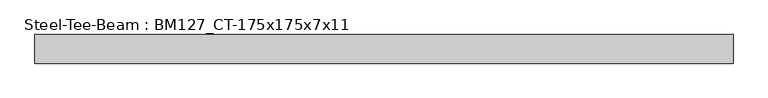
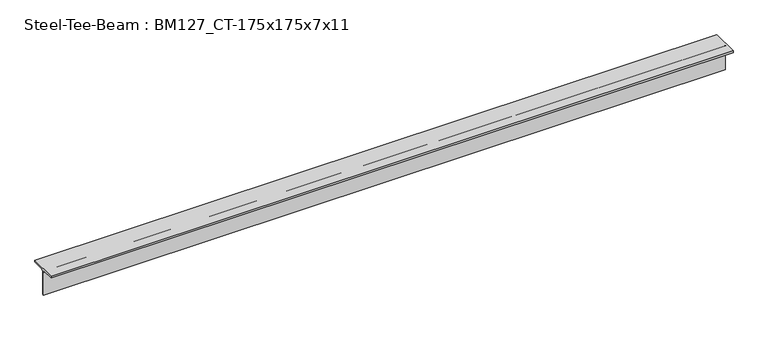
"""IFC4 building model written with IfcOpenShell, lengths in millimetres: beam geometry, Steel-Tee-Beam : BM127_CT-175x175x7x11."""

import ifcopenshell
import ifcopenshell.guid

model = None  # the IFC model being written
_history = None  # IfcOwnerHistory: only IFC2X3 demands one
_inside = {}  # id of a spatial element -> (the spatial element, [elements in it])
_under = {}  # id of a project, library or spatial element -> (it, [spatial elements below it])
_declared = {}  # id of a project -> (the project, [libraries it declares])
_typed = {}  # id of a type object -> (the type object, [elements of that type])
_made_of = {}  # id of a material, layer set ... -> (it, [elements and type objects made of it])


def new_model(schema):
    """Start an empty IFC model of exactly this schema.

    Asked for "IFC4X3", IfcOpenShell would pick the latest addendum, in which some entities
    have other attributes; the version numbers below select the first issue.
    IFC2X3 requires an IfcOwnerHistory on every rooted entity: one is made here for all.
    """
    global model, _history
    if schema == "IFC4X3":
        model = ifcopenshell.file(schema_version=(4, 3, 0, 0))
    else:
        model = ifcopenshell.file(schema=schema)
    _inside.clear()
    _under.clear()
    _declared.clear()
    _typed.clear()
    _made_of.clear()
    _history = None
    if model.schema == "IFC2X3":
        org = make("IfcOrganization", Name="unknown")
        user = make(
            "IfcPersonAndOrganization",
            ThePerson=make("IfcPerson", FamilyName="unknown"),
            TheOrganization=org,
        )
        app = make(
            "IfcApplication",
            ApplicationDeveloper=org,
            Version="unknown",
            ApplicationFullName="unknown",
            ApplicationIdentifier="unknown",
        )
        _history = make(
            "IfcOwnerHistory",
            OwningUser=user,
            OwningApplication=app,
            ChangeAction="ADDED",
            CreationDate=0,
        )
    return model


def make(cls, **values):
    """One entity of the class cls with the attributes given. An attribute that is None is left unset."""
    return model.create_entity(
        cls, **{name: value for name, value in values.items() if value is not None}
    )


def rooted(cls, **values):
    """An entity with a GlobalId (a new one), such as an element, a storey or a relation."""
    return make(cls, GlobalId=ifcopenshell.guid.new(), OwnerHistory=_history, **values)


def si_unit(unit_type, name, prefix=None):
    """IfcSIUnit, for example si_unit("LENGTHUNIT", "METRE", prefix="MILLI")."""
    return make("IfcSIUnit", UnitType=unit_type, Prefix=prefix, Name=name)


def assignment(units):
    """IfcUnitAssignment: the units of a project."""
    return None if units is None else make("IfcUnitAssignment", Units=units)


def point(xyz):
    """IfcCartesianPoint."""
    return None if xyz is None else make("IfcCartesianPoint", Coordinates=xyz)


def direction(xyz):
    """IfcDirection."""
    return None if xyz is None else make("IfcDirection", DirectionRatios=xyz)


def frame(location, z_axis=None, x_axis=None):
    """IfcAxis2Placement3D, a coordinate frame: its origin and axes. An axis left out is left unset."""
    return make(
        "IfcAxis2Placement3D",
        Location=point(location),
        Axis=direction(z_axis),
        RefDirection=direction(x_axis),
    )


def frame_2d(location, x_axis=None):
    """IfcAxis2Placement2D, a coordinate frame in the plane: its origin and x axis."""
    return make(
        "IfcAxis2Placement2D", Location=point(location), RefDirection=direction(x_axis)
    )


def origin():
    """The frame at (0, 0, 0) with its axes left unset."""
    return frame((0.0, 0.0, 0.0))


def place(relative_to, where):
    """IfcLocalPlacement: puts the frame where relative to a parent placement (None: the world)."""
    return make(
        "IfcLocalPlacement", PlacementRelTo=relative_to, RelativePlacement=where
    )


def context(
    kind, dimensions, precision=None, world=None, true_north=None, identifier=None
):
    """IfcGeometricRepresentationContext, for example the 3D "Model" context."""
    return make(
        "IfcGeometricRepresentationContext",
        ContextIdentifier=identifier,
        ContextType=kind,
        CoordinateSpaceDimension=dimensions,
        Precision=precision,
        WorldCoordinateSystem=world,
        TrueNorth=true_north,
    )


def project(units=None, contexts=None):
    """IfcProject with its units and contexts."""
    return rooted(
        "IfcProject",
        Name="project",
        RepresentationContexts=contexts,
        UnitsInContext=assignment(units),
    )


def spatial(cls, under=None, at=None, **own):
    """A site, building, storey or space (cls), placed at a placement, below another one or the project."""
    s = rooted(cls, ObjectPlacement=at, **own)
    if under is not None:
        _under.setdefault(under.id(), (under, []))[1].append(s)
    return s


def polyline(points):
    """IfcPolyline through the points."""
    return make("IfcPolyline", Points=[point(p) for p in points])


def circle_curve(where, radius):
    """IfcCircle in the frame where."""
    return make("IfcCircle", Position=where, Radius=radius)


def trimmed(basis, trim1, trim2, sense, master):
    """IfcTrimmedCurve: the piece of a basis curve between two trims."""
    return make(
        "IfcTrimmedCurve",
        BasisCurve=basis,
        Trim1=trim1,
        Trim2=trim2,
        SenseAgreement=sense,
        MasterRepresentation=master,
    )


def segment(curve, same_sense, transition):
    """IfcCompositeCurveSegment."""
    return make(
        "IfcCompositeCurveSegment",
        Transition=transition,
        SameSense=same_sense,
        ParentCurve=curve,
    )


def composite_curve(segments, self_intersect=None):
    """IfcCompositeCurve: segments joined end to end."""
    return make("IfcCompositeCurve", Segments=segments, SelfIntersect=self_intersect)


def outline(outer, holes=None, kind="AREA"):
    """IfcArbitraryClosedProfileDef: a profile drawn as a closed curve; with holes, ...WithVoids."""
    if holes is None:
        return make("IfcArbitraryClosedProfileDef", ProfileType=kind, OuterCurve=outer)
    return make(
        "IfcArbitraryProfileDefWithVoids",
        ProfileType=kind,
        OuterCurve=outer,
        InnerCurves=holes,
    )


def extrude(swept, where, along, depth):
    """IfcExtrudedAreaSolid: the profile swept, set in the frame where, extruded along a direction by depth."""
    return make(
        "IfcExtrudedAreaSolid",
        SweptArea=swept,
        Position=where,
        ExtrudedDirection=direction(along),
        Depth=depth,
    )


def shape(context_of_items, identifier, shape_type, items):
    """IfcShapeRepresentation: the items that make up one representation, for example the "Body"."""
    return make(
        "IfcShapeRepresentation",
        ContextOfItems=context_of_items,
        RepresentationIdentifier=identifier,
        RepresentationType=shape_type,
        Items=items,
    )


def source(mapping_origin, context_of_items, identifier, shape_type, items):
    """IfcRepresentationMap: a shape defined once, which mapped items show again and again."""
    return make(
        "IfcRepresentationMap",
        MappingOrigin=mapping_origin,
        MappedRepresentation=shape(context_of_items, identifier, shape_type, items),
    )


def transform(
    local_origin,
    x_axis=None,
    y_axis=None,
    z_axis=None,
    scale=None,
    scale2=None,
    scale3=None,
    uniform=True,
):
    """IfcCartesianTransformationOperator3D, or its non-uniform kind. x_axis, y_axis, z_axis: its Axis1, 2, 3."""
    if uniform:
        return make(
            "IfcCartesianTransformationOperator3D",
            Axis1=direction(x_axis),
            Axis2=direction(y_axis),
            LocalOrigin=point(local_origin),
            Scale=scale,
            Axis3=direction(z_axis),
        )
    return make(
        "IfcCartesianTransformationOperator3DnonUniform",
        Axis1=direction(x_axis),
        Axis2=direction(y_axis),
        LocalOrigin=point(local_origin),
        Scale=scale,
        Axis3=direction(z_axis),
        Scale2=scale2,
        Scale3=scale3,
    )


def mapped(mapping_source, mapping_target):
    """IfcMappedItem: shows the shape of a source again, moved by a transform."""
    return make(
        "IfcMappedItem", MappingSource=mapping_source, MappingTarget=mapping_target
    )


def made_of(thing, what):
    """Note that an element or type object is made of a material, layer set ...; save() writes the relation."""
    if what is not None:
        _made_of.setdefault(what.id(), (what, []))[1].append(thing)
    return thing


def element(
    cls,
    number,
    at=None,
    inside=None,
    cuts=None,
    type_object=None,
    material=None,
    context=None,
    identifier="Body",
    shape_type=None,
    held_by="IfcProductDefinitionShape",
    body=None,
    shapes=None,
    **own,
):
    """One element of the class cls, such as IfcWall. Its Tag is "e" and its number.

    at: its placement. inside: the storey or other place that contains it. cuts: it is an
    opening in that element (IfcRelVoidsElement). A single representation is given by context,
    identifier, shape_type and body (its items); several are given by shapes. held_by: the class
    of the entity that holds the representations. save() writes the other relations.
    """
    e = rooted(cls, Tag="e%d" % number, ObjectPlacement=at, **own)
    if body is not None:
        shapes = [shape(context, identifier, shape_type, body)]
    if shapes is not None:
        e.Representation = make(held_by, Representations=shapes)
    if inside is not None:
        _inside.setdefault(inside.id(), (inside, []))[1].append(e)
    if cuts is not None:
        rooted(
            "IfcRelVoidsElement", RelatingBuildingElement=cuts, RelatedOpeningElement=e
        )
    if type_object is not None:
        _typed.setdefault(type_object.id(), (type_object, []))[1].append(e)
    return made_of(e, material)


def aggregate(whole, parts):
    """IfcRelAggregates: a whole, such as a stair, and the parts it consists of."""
    return rooted("IfcRelAggregates", RelatingObject=whole, RelatedObjects=parts)


def save(model, path):
    """Write the relations noted so far, then the file.

    IfcRelAggregates (storeys below a building ...), IfcRelContainedInSpatialStructure (elements
    in a storey), IfcRelDefinesByType, IfcRelAssociatesMaterial and IfcRelDeclares: one each for
    every whole, place, type object, material and project.
    """
    for whole, parts in _under.values():
        aggregate(whole, parts)
    for where, things in _inside.values():
        rooted(
            "IfcRelContainedInSpatialStructure",
            RelatedElements=things,
            RelatingStructure=where,
        )
    for kind, things in _typed.values():
        rooted("IfcRelDefinesByType", RelatedObjects=things, RelatingType=kind)
    for what, things in _made_of.values():
        rooted("IfcRelAssociatesMaterial", RelatedObjects=things, RelatingMaterial=what)
    for by, libraries in _declared.values():
        rooted("IfcRelDeclares", RelatingContext=by, RelatedDefinitions=libraries)
    model.write(path)


def steel_tee_beam_bm127_ct_175x175x7x11_f7a1ba5a(model_context):
    return source(origin(), model_context, "Body", "SweptSolid", [
        extrude(outline(composite_curve([segment(polyline([(-87.5, 87.5), (87.5, 87.5), (87.5, 76.5), (17.5, 76.5)]), True, "CONTINUOUS"), segment(trimmed(circle_curve(frame_2d((17.5, 62.5)), 14.0), [point((17.5, 76.5))], [point((3.5, 62.5))], True, "CARTESIAN"), True, "CONTINUOUS"), segment(polyline([(3.5, 62.5), (3.5, -87.5), (-3.5, -87.5), (-3.5, 62.5)]), True, "CONTINUOUS"), segment(trimmed(circle_curve(frame_2d((-17.5, 62.5)), 14.0), [point((-3.5, 62.5))], [point((-17.5, 76.5))], True, "CARTESIAN"), True, "CONTINUOUS"), segment(polyline([(-17.5, 76.5), (-87.5, 76.5), (-87.5, 87.5)]), True, "CONTINUOUS")], self_intersect=False)), frame((-2078.5248279, 0.0, 0.0), z_axis=(1.0, 0.0, 0.0), x_axis=(0.0, 1.0, 0.0)), (0.0, 0.0, 1.0), 4262.7315887),
    ])


if __name__ == "__main__":
    model = new_model("IFC4")
    model_context = context("Model", 3, world=origin())
    ifc_project = project(units=[si_unit("LENGTHUNIT", "METRE", prefix="MILLI")], contexts=[model_context])
    site = spatial("IfcSite", under=ifc_project)
    building = spatial("IfcBuilding", under=site)
    placement = place(None, origin())
    steel_tee_beam_bm127_ct_175x175x7x11_shape = steel_tee_beam_bm127_ct_175x175x7x11_f7a1ba5a(model_context)
    element("IfcBeam", 1, ObjectType="Steel-Tee-Beam : BM127_CT-175x175x7x11", at=placement, inside=building, context=model_context, shape_type="MappedRepresentation", body=[
        mapped(steel_tee_beam_bm127_ct_175x175x7x11_shape, transform((0.0, 0.0, 0.0), x_axis=(1.0, 0.0, 0.0), y_axis=(0.0, 1.0, 0.0), z_axis=(0.0, 0.0, 1.0))),
    ])
    save(model, "model.ifc")

# Revit data of these elements
# Type "Steel-Tee-Beam : BM127_CT-175x175x7x11"
#   Section Area = 31.57 cm²
#   Mass per Unit Length = 24.80 kg/m
#   Length [instance default] = 1524 mm
#   bf = 175 mm
#   d = 175 mm
#   k = 25 mm
#   kr = 14 mm
#   tf = 11 mm
#   tw = 7 mm
#   hec_material4 [instance default] = none
#   hec_material3 [instance default] = none
#   hec_material2 [instance default] = none
#   hec_material1 [instance default] = none
#   Structural Material [instance default] = Steel, 45-345
#   Assembly Code = ""
# Element 1 (IfcBeam, "Steel-Tee-Beam : BM127_CT-175x175x7x11")
#   hec_material3 = F01AC000-00002_Building/Shelter Fire Proofing Work_Intumescent Coating Type_1 hr. rating (UL 1709))
#   hec_material1 = S03AA029-00001_Main Steel Structure Erection Work_Shelter/Building_Light Steel
#   Structural Material = S01AA003-00001_Main Steel Structure Fabrication Work_Shelter/Building_Light Steel - Standard
#   Materials on its faces: "S01AA003-00001_Main Steel Structure Fabrication Work_Shelter/Building_Light Steel - Standard"
# Materials
#   "Steel, 45-345": class "Metal", colour RGB 189 187 185, transparency 0, Description = "Steel 345 MPa", Cost = 0
#   "S01AA003-00001_Main Steel Structure Fabrication Work_Shelter/Building_Light Steel - Standard": class "Metal", colour RGB 120 120 120, transparency 0, Comments = "(30KG/M>Weight)", Description = "Structural steel 50ksi", W00) Work Master Code = "S01AA003-00001", W01) Work Master_Lv1 = "Main Steel Structure Fabrication Work", W02) Work Master_Lv2 = "Shelter/Building", W03) Work Master_Spec.1 = "Light Steel - Standard (30KG/M>Weight)", Cost = 0
#   "F01AC000-00002_Building/Shelter Fire Proofing Work_Intumescent Coating Type_1 hr. rating (UL 1709))": class "Metal", colour RGB 255 128 128, transparency 0, Description = "Paint finished steel", W00) Work Master Code = "F01AC000-00002", W01) Work Master_Lv1 = "Building/Shelter Fire Proofing Work", W02) Work Master_Lv2 = "Intumescent Coating Type", W03) Work Master_Spec.1 = "1 hr. rating (UL 1709)", Cost = 0
#   "S03AA029-00001_Main Steel Structure Erection Work_Shelter/Building_Light Steel": class "Metal", colour RGB 120 120 120, transparency 0, Comments = "(30KG/M>Weight)", Description = "Structural steel 50ksi", W00) Work Master Code = "S03AA029-00001", W01) Work Master_Lv1 = "Main Steel Structure Erection Work", W02) Work Master_Lv2 = "Shelter/Building", W03) Work Master_Spec.1 = "Light Steel (30KG/M>Weight)", Cost = 0
